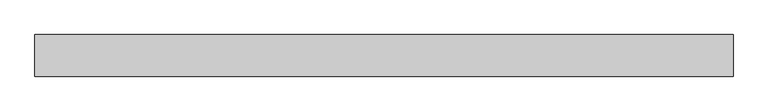
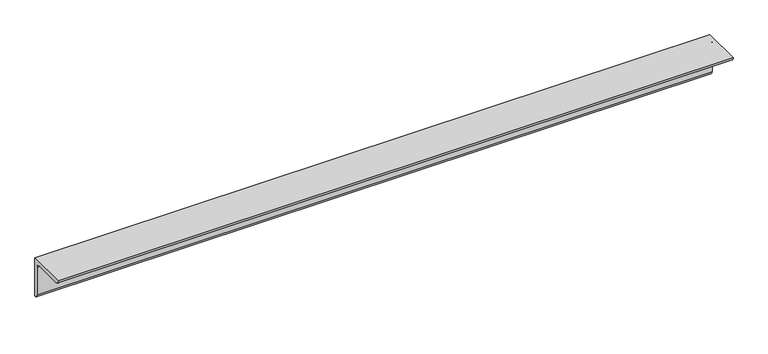
"""IFC4 building model written with IfcOpenShell, lengths in millimetres: member geometry, 0912_Steel Framing_L-KSD3502 : H_SB_AR_S03_L-130x130x12_HBR3."""

import ifcopenshell
import ifcopenshell.guid

model = None  # the IFC model being written
_history = None  # IfcOwnerHistory: only IFC2X3 demands one
_inside = {}  # id of a spatial element -> (the spatial element, [elements in it])
_under = {}  # id of a project, library or spatial element -> (it, [spatial elements below it])
_declared = {}  # id of a project -> (the project, [libraries it declares])
_typed = {}  # id of a type object -> (the type object, [elements of that type])
_made_of = {}  # id of a material, layer set ... -> (it, [elements and type objects made of it])


def new_model(schema):
    """Start an empty IFC model of exactly this schema.

    Asked for "IFC4X3", IfcOpenShell would pick the latest addendum, in which some entities
    have other attributes; the version numbers below select the first issue.
    IFC2X3 requires an IfcOwnerHistory on every rooted entity: one is made here for all.
    """
    global model, _history
    if schema == "IFC4X3":
        model = ifcopenshell.file(schema_version=(4, 3, 0, 0))
    else:
        model = ifcopenshell.file(schema=schema)
    _inside.clear()
    _under.clear()
    _declared.clear()
    _typed.clear()
    _made_of.clear()
    _history = None
    if model.schema == "IFC2X3":
        org = make("IfcOrganization", Name="unknown")
        user = make(
            "IfcPersonAndOrganization",
            ThePerson=make("IfcPerson", FamilyName="unknown"),
            TheOrganization=org,
        )
        app = make(
            "IfcApplication",
            ApplicationDeveloper=org,
            Version="unknown",
            ApplicationFullName="unknown",
            ApplicationIdentifier="unknown",
        )
        _history = make(
            "IfcOwnerHistory",
            OwningUser=user,
            OwningApplication=app,
            ChangeAction="ADDED",
            CreationDate=0,
        )
    return model


def make(cls, **values):
    """One entity of the class cls with the attributes given. An attribute that is None is left unset."""
    return model.create_entity(
        cls, **{name: value for name, value in values.items() if value is not None}
    )


def rooted(cls, **values):
    """An entity with a GlobalId (a new one), such as an element, a storey or a relation."""
    return make(cls, GlobalId=ifcopenshell.guid.new(), OwnerHistory=_history, **values)


def si_unit(unit_type, name, prefix=None):
    """IfcSIUnit, for example si_unit("LENGTHUNIT", "METRE", prefix="MILLI")."""
    return make("IfcSIUnit", UnitType=unit_type, Prefix=prefix, Name=name)


def assignment(units):
    """IfcUnitAssignment: the units of a project."""
    return None if units is None else make("IfcUnitAssignment", Units=units)


def point(xyz):
    """IfcCartesianPoint."""
    return None if xyz is None else make("IfcCartesianPoint", Coordinates=xyz)


def direction(xyz):
    """IfcDirection."""
    return None if xyz is None else make("IfcDirection", DirectionRatios=xyz)


def frame(location, z_axis=None, x_axis=None):
    """IfcAxis2Placement3D, a coordinate frame: its origin and axes. An axis left out is left unset."""
    return make(
        "IfcAxis2Placement3D",
        Location=point(location),
        Axis=direction(z_axis),
        RefDirection=direction(x_axis),
    )


def frame_2d(location, x_axis=None):
    """IfcAxis2Placement2D, a coordinate frame in the plane: its origin and x axis."""
    return make(
        "IfcAxis2Placement2D", Location=point(location), RefDirection=direction(x_axis)
    )


def origin():
    """The frame at (0, 0, 0) with its axes left unset."""
    return frame((0.0, 0.0, 0.0))


def place(relative_to, where):
    """IfcLocalPlacement: puts the frame where relative to a parent placement (None: the world)."""
    return make(
        "IfcLocalPlacement", PlacementRelTo=relative_to, RelativePlacement=where
    )


def context(
    kind, dimensions, precision=None, world=None, true_north=None, identifier=None
):
    """IfcGeometricRepresentationContext, for example the 3D "Model" context."""
    return make(
        "IfcGeometricRepresentationContext",
        ContextIdentifier=identifier,
        ContextType=kind,
        CoordinateSpaceDimension=dimensions,
        Precision=precision,
        WorldCoordinateSystem=world,
        TrueNorth=true_north,
    )


def project(units=None, contexts=None):
    """IfcProject with its units and contexts."""
    return rooted(
        "IfcProject",
        Name="project",
        RepresentationContexts=contexts,
        UnitsInContext=assignment(units),
    )


def spatial(cls, under=None, at=None, **own):
    """A site, building, storey or space (cls), placed at a placement, below another one or the project."""
    s = rooted(cls, ObjectPlacement=at, **own)
    if under is not None:
        _under.setdefault(under.id(), (under, []))[1].append(s)
    return s


def polyline(points):
    """IfcPolyline through the points."""
    return make("IfcPolyline", Points=[point(p) for p in points])


def circle_curve(where, radius):
    """IfcCircle in the frame where."""
    return make("IfcCircle", Position=where, Radius=radius)


def trimmed(basis, trim1, trim2, sense, master):
    """IfcTrimmedCurve: the piece of a basis curve between two trims."""
    return make(
        "IfcTrimmedCurve",
        BasisCurve=basis,
        Trim1=trim1,
        Trim2=trim2,
        SenseAgreement=sense,
        MasterRepresentation=master,
    )


def segment(curve, same_sense, transition):
    """IfcCompositeCurveSegment."""
    return make(
        "IfcCompositeCurveSegment",
        Transition=transition,
        SameSense=same_sense,
        ParentCurve=curve,
    )


def composite_curve(segments, self_intersect=None):
    """IfcCompositeCurve: segments joined end to end."""
    return make("IfcCompositeCurve", Segments=segments, SelfIntersect=self_intersect)


def outline(outer, holes=None, kind="AREA"):
    """IfcArbitraryClosedProfileDef: a profile drawn as a closed curve; with holes, ...WithVoids."""
    if holes is None:
        return make("IfcArbitraryClosedProfileDef", ProfileType=kind, OuterCurve=outer)
    return make(
        "IfcArbitraryProfileDefWithVoids",
        ProfileType=kind,
        OuterCurve=outer,
        InnerCurves=holes,
    )


def extrude(swept, where, along, depth):
    """IfcExtrudedAreaSolid: the profile swept, set in the frame where, extruded along a direction by depth."""
    return make(
        "IfcExtrudedAreaSolid",
        SweptArea=swept,
        Position=where,
        ExtrudedDirection=direction(along),
        Depth=depth,
    )


def shape(context_of_items, identifier, shape_type, items):
    """IfcShapeRepresentation: the items that make up one representation, for example the "Body"."""
    return make(
        "IfcShapeRepresentation",
        ContextOfItems=context_of_items,
        RepresentationIdentifier=identifier,
        RepresentationType=shape_type,
        Items=items,
    )


def source(mapping_origin, context_of_items, identifier, shape_type, items):
    """IfcRepresentationMap: a shape defined once, which mapped items show again and again."""
    return make(
        "IfcRepresentationMap",
        MappingOrigin=mapping_origin,
        MappedRepresentation=shape(context_of_items, identifier, shape_type, items),
    )


def transform(
    local_origin,
    x_axis=None,
    y_axis=None,
    z_axis=None,
    scale=None,
    scale2=None,
    scale3=None,
    uniform=True,
):
    """IfcCartesianTransformationOperator3D, or its non-uniform kind. x_axis, y_axis, z_axis: its Axis1, 2, 3."""
    if uniform:
        return make(
            "IfcCartesianTransformationOperator3D",
            Axis1=direction(x_axis),
            Axis2=direction(y_axis),
            LocalOrigin=point(local_origin),
            Scale=scale,
            Axis3=direction(z_axis),
        )
    return make(
        "IfcCartesianTransformationOperator3DnonUniform",
        Axis1=direction(x_axis),
        Axis2=direction(y_axis),
        LocalOrigin=point(local_origin),
        Scale=scale,
        Axis3=direction(z_axis),
        Scale2=scale2,
        Scale3=scale3,
    )


def mapped(mapping_source, mapping_target):
    """IfcMappedItem: shows the shape of a source again, moved by a transform."""
    return make(
        "IfcMappedItem", MappingSource=mapping_source, MappingTarget=mapping_target
    )


def made_of(thing, what):
    """Note that an element or type object is made of a material, layer set ...; save() writes the relation."""
    if what is not None:
        _made_of.setdefault(what.id(), (what, []))[1].append(thing)
    return thing


def element(
    cls,
    number,
    at=None,
    inside=None,
    cuts=None,
    type_object=None,
    material=None,
    context=None,
    identifier="Body",
    shape_type=None,
    held_by="IfcProductDefinitionShape",
    body=None,
    shapes=None,
    **own,
):
    """One element of the class cls, such as IfcWall. Its Tag is "e" and its number.

    at: its placement. inside: the storey or other place that contains it. cuts: it is an
    opening in that element (IfcRelVoidsElement). A single representation is given by context,
    identifier, shape_type and body (its items); several are given by shapes. held_by: the class
    of the entity that holds the representations. save() writes the other relations.
    """
    e = rooted(cls, Tag="e%d" % number, ObjectPlacement=at, **own)
    if body is not None:
        shapes = [shape(context, identifier, shape_type, body)]
    if shapes is not None:
        e.Representation = make(held_by, Representations=shapes)
    if inside is not None:
        _inside.setdefault(inside.id(), (inside, []))[1].append(e)
    if cuts is not None:
        rooted(
            "IfcRelVoidsElement", RelatingBuildingElement=cuts, RelatedOpeningElement=e
        )
    if type_object is not None:
        _typed.setdefault(type_object.id(), (type_object, []))[1].append(e)
    return made_of(e, material)


def aggregate(whole, parts):
    """IfcRelAggregates: a whole, such as a stair, and the parts it consists of."""
    return rooted("IfcRelAggregates", RelatingObject=whole, RelatedObjects=parts)


def save(model, path):
    """Write the relations noted so far, then the file.

    IfcRelAggregates (storeys below a building ...), IfcRelContainedInSpatialStructure (elements
    in a storey), IfcRelDefinesByType, IfcRelAssociatesMaterial and IfcRelDeclares: one each for
    every whole, place, type object, material and project.
    """
    for whole, parts in _under.values():
        aggregate(whole, parts)
    for where, things in _inside.values():
        rooted(
            "IfcRelContainedInSpatialStructure",
            RelatedElements=things,
            RelatingStructure=where,
        )
    for kind, things in _typed.values():
        rooted("IfcRelDefinesByType", RelatedObjects=things, RelatingType=kind)
    for what, things in _made_of.values():
        rooted("IfcRelAssociatesMaterial", RelatedObjects=things, RelatingMaterial=what)
    for by, libraries in _declared.values():
        rooted("IfcRelDeclares", RelatingContext=by, RelatedDefinitions=libraries)
    model.write(path)


def member_70962aff(model_context):
    return source(origin(), model_context, "Body", "SweptSolid", [
        extrude(outline(composite_curve([segment(polyline([(36.4, 36.4), (36.4, -93.6)]), True, "CONTINUOUS"), segment(trimmed(circle_curve(frame_2d((36.4, -81.6)), 12.0), [point((36.4, -93.6))], [point((24.4, -81.6))], False, "CARTESIAN"), True, "CONTINUOUS"), segment(polyline([(24.4, -81.6), (24.4, 12.4)]), True, "CONTINUOUS"), segment(trimmed(circle_curve(frame_2d((12.4, 12.4)), 12.0), [point((24.4, 12.4))], [point((12.4, 24.4))], True, "CARTESIAN"), True, "CONTINUOUS"), segment(polyline([(12.4, 24.4), (-81.6, 24.4)]), True, "CONTINUOUS"), segment(trimmed(circle_curve(frame_2d((-81.6, 36.4)), 12.0), [point((-81.6, 24.4))], [point((-93.6, 36.4))], False, "CARTESIAN"), True, "CONTINUOUS"), segment(polyline([(-93.6, 36.4), (36.4, 36.4)]), True, "CONTINUOUS")], self_intersect=False)), frame((-995.2380761, 0.0, 0.0), z_axis=(1.0, 0.0, 0.0), x_axis=(0.0, 1.0, 0.0)), (0.0, 0.0, 1.0), 2181.7834935),
    ])


if __name__ == "__main__":
    model = new_model("IFC4")
    model_context = context("Model", 3, world=origin())
    ifc_project = project(units=[si_unit("LENGTHUNIT", "METRE", prefix="MILLI")], contexts=[model_context])
    site = spatial("IfcSite", under=ifc_project)
    building = spatial("IfcBuilding", under=site)
    placement = place(None, origin())
    member_shape = member_70962aff(model_context)
    element("IfcMember", 1, ObjectType="0912_Steel Framing_L-KSD3502 : H_SB_AR_S03_L-130x130x12_HBR3", at=placement, inside=building, context=model_context, shape_type="MappedRepresentation", body=[
        mapped(member_shape, transform((0.0, 0.0, 0.0), x_axis=(1.0, 0.0, 0.0), y_axis=(0.0, 1.0, 0.0), z_axis=(0.0, 0.0, 1.0))),
    ])
    save(model, "model.ifc")

# Revit data of these elements
# Type "0912_Steel Framing_L-KSD3502 : H_SB_AR_S03_L-130x130x12_HBR3"
#   k = 25 mm
#   Perimeter = 0.52 m²/m
#   Nominal Weight = 23.40 kgf/m
#   Length [instance default] = 1000 mm
#   b = 130 mm
#   d = 130 mm
#   t = 12 mm
#   x = 36.4 mm
#   y = 36.4 mm
#   A = 2976.00 m²
#   Structural Material [instance default] = Steel, 45-345
# Element 1 (IfcMember, "0912_Steel Framing_L-KSD3502 : H_SB_AR_S03_L-130x130x12_HBR3")
#   Materials on its faces: "Steel, 45-345"
# Materials
#   "Steel, 45-345": class "Metal", colour RGB 189 187 185, transparency 0, Description = "Steel 345 MPa", Cost = 0
